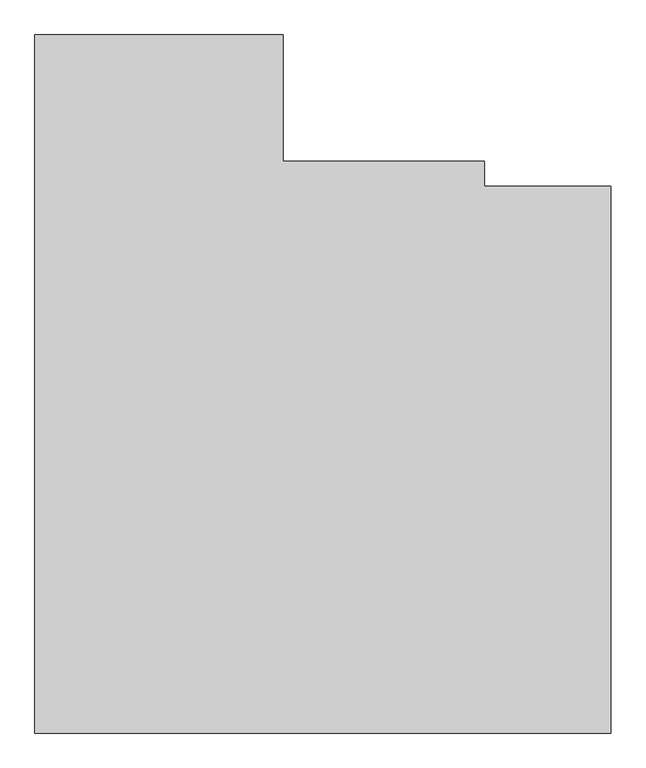
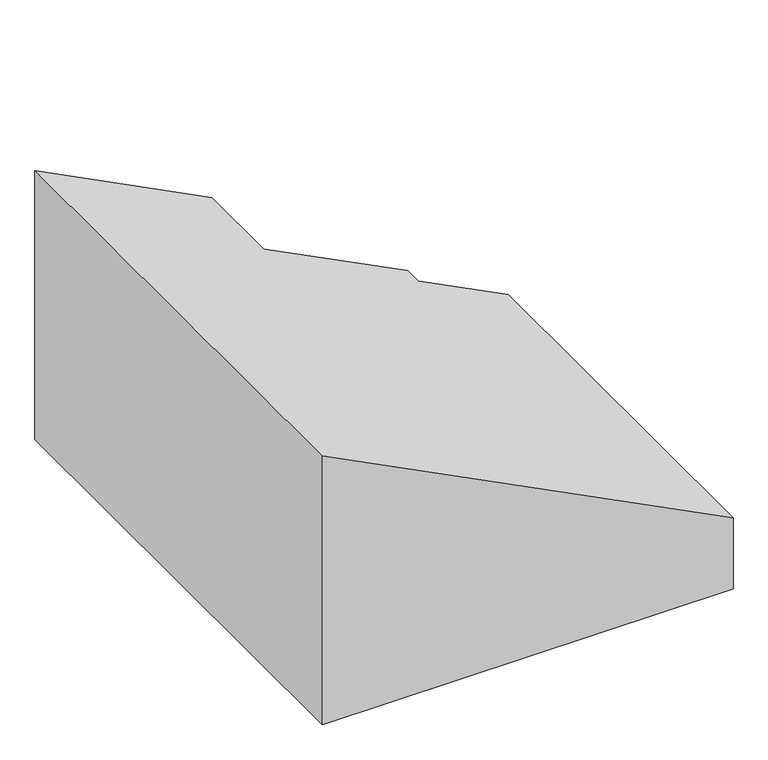
"""IFC4 building model written with IfcOpenShell, lengths in millimetres: proxy geometry, 0_3d."""

from ifc_helpers import new_model, si_unit, origin, place, context, project, spatial, faceted_brep, source, transform, mapped, element, save


def generic_models_0269b9af(model_context):
    return source(origin(), model_context, "Body", "Brep", [
        faceted_brep([(4680.0, 4440.2642941, 853.3339073), (3655.0, 4440.2642941, 1375.5974931), (3655.0, 4645.0, 1375.5974931), (2015.3981634, 4645.0, 2211.0163558), (2015.0, 5670.0, 2211.2192302), (0.0, 5670.0, 3237.913011), (0.0, 0.0, 3237.913011), (4680.0, 0.0, 853.3339073), (2015.0, 5670.0, 0.0), (0.0, 5670.0, 0.0), (2015.3981634, 4645.0, 0.0), (3655.0, 4645.0, 0.0), (3655.0, 4440.2642941, 0.0), (4680.0, 4440.2642941, 0.0), (4680.0, 0.0, 0.0), (0.0, 0.0, 0.0)], [[[0, 1, 2, 3, 4, 5, 6, 7]], [[5, 4, 8, 9]], [[4, 3, 10, 8]], [[3, 2, 11, 10]], [[2, 1, 12, 11]], [[1, 0, 13, 12]], [[0, 7, 14, 13]], [[7, 6, 15, 14]], [[9, 15, 6, 5]], [[11, 12, 13, 14, 15, 9, 8, 10]]]),
    ])


if __name__ == "__main__":
    model = new_model("IFC4")
    model_context = context("Model", 3, world=origin())
    ifc_project = project(units=[si_unit("LENGTHUNIT", "METRE", prefix="MILLI")], contexts=[model_context])
    site = spatial("IfcSite", under=ifc_project)
    building = spatial("IfcBuilding", under=site)
    placement = place(None, origin())
    generic_models_shape = generic_models_0269b9af(model_context)
    element("IfcBuildingElementProxy", 1, Name="0_3d", ObjectType="0_3d", at=placement, inside=building, context=model_context, shape_type="MappedRepresentation", body=[
        mapped(generic_models_shape, transform((0.0, 0.0, 0.0), x_axis=(1.0, 0.0, 0.0), y_axis=(0.0, 1.0, 0.0), z_axis=(0.0, 0.0, 1.0))),
    ])
    save(model, "model.ifc")

# Revit data of these elements
# Element 1 (IfcBuildingElementProxy, "0_3d")
#   Materials on its faces: "*1"
# Materials
#   "*1": class "Unassigned", colour RGB 175 175 175, transparency 0
